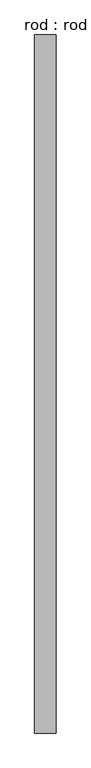
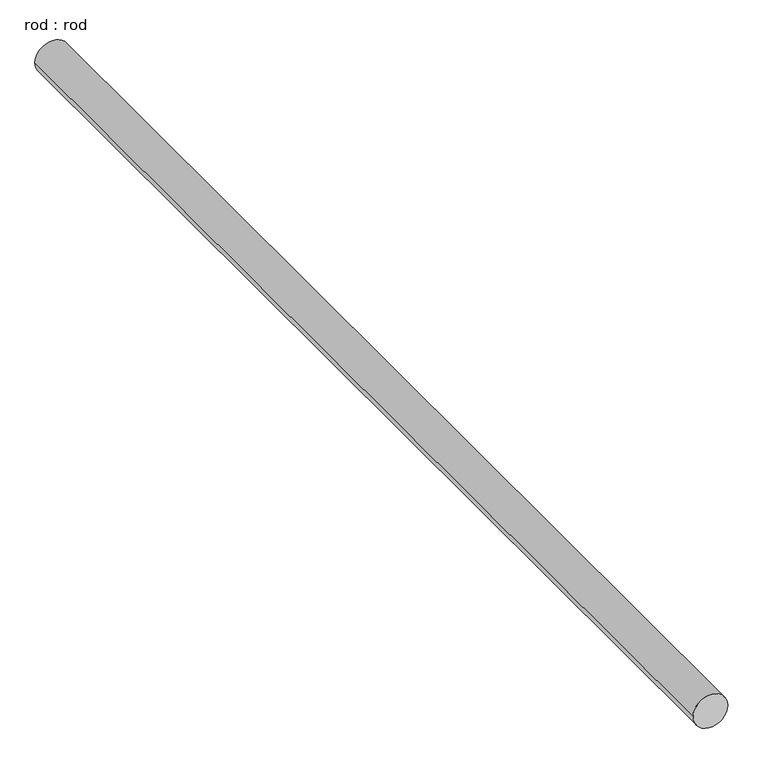
"""IFC4 building model written with IfcOpenShell, lengths in millimetres: proxy geometry, rod : rod."""

from ifc_helpers import new_model, si_unit, point, frame, frame_2d, origin, place, context, project, spatial, circle_curve, trimmed, segment, composite_curve, outline, extrude, source, transform, mapped, element, save


def rod_rod_c0ad713d(model_context):
    return source(origin(), model_context, "Body", "SweptSolid", [
        extrude(outline(composite_curve([segment(trimmed(circle_curve(frame_2d((0.0108462, 0.0)), 200.0), [point((0.0108462, 200.0))], [point((0.0108462, -200.0))], False, "CARTESIAN"), True, "CONTINUOUS"), segment(trimmed(circle_curve(frame_2d((0.0108462, 0.0)), 200.0), [point((0.0108462, -200.0))], [point((0.0108462, 200.0))], False, "CARTESIAN"), True, "CONTINUOUS")], self_intersect=False)), frame((0.0, -2478.6999561, 0.0), z_axis=(0.0, 1.0, 0.0), x_axis=(0.0, 0.0, 1.0)), (0.0, 0.0, 1.0), 13142.8571429),
    ])


if __name__ == "__main__":
    model = new_model("IFC4")
    model_context = context("Model", 3, world=origin())
    ifc_project = project(units=[si_unit("LENGTHUNIT", "METRE", prefix="MILLI")], contexts=[model_context])
    site = spatial("IfcSite", under=ifc_project)
    building = spatial("IfcBuilding", under=site)
    placement = place(None, origin())
    rod_rod_shape = rod_rod_c0ad713d(model_context)
    element("IfcBuildingElementProxy", 1, Name="rod : rod", ObjectType="rod : rod", at=placement, inside=building, context=model_context, shape_type="MappedRepresentation", body=[
        mapped(rod_rod_shape, transform((0.0, 0.0, 0.0), x_axis=(1.0, 0.0, 0.0), y_axis=(0.0, 1.0, 0.0), z_axis=(0.0, 0.0, 1.0))),
    ])
    save(model, "model.ifc")

# Revit data of these elements
# Type "rod : rod"
#   Default Elevation = 0
